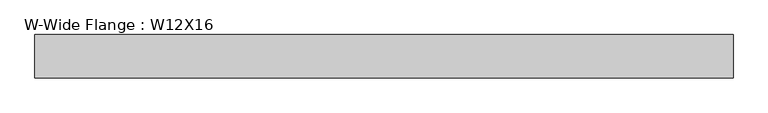
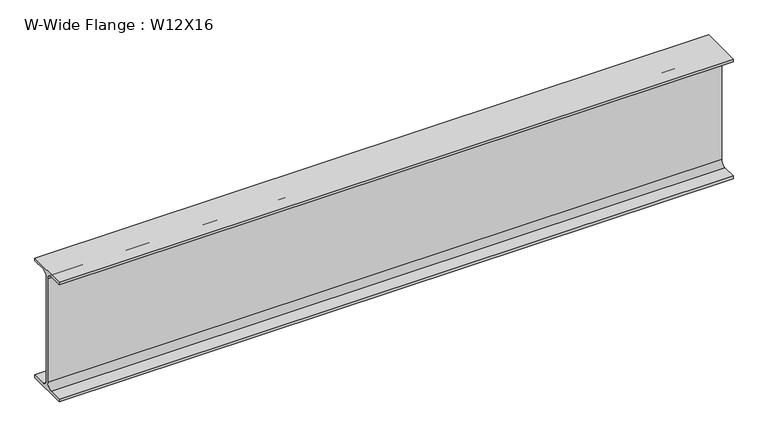
"""IFC4 building model written with IfcOpenShell, lengths in millimetres: beam geometry, W-Wide Flange : W12X16."""

from ifc_helpers import new_model, si_unit, point, frame, frame_2d, origin, place, context, project, spatial, polyline, circle_curve, trimmed, segment, composite_curve, outline, extrude, source, transform, mapped, element, save


def w_wide_flange_w12x16_6f895092(model_context):
    return source(origin(), model_context, "Body", "SweptSolid", [
        extrude(outline(composite_curve([segment(polyline([(50.673, -145.669), (50.673, -152.4), (-50.673, -152.4), (-50.673, -145.669), (-16.7005, -145.669)]), True, "CONTINUOUS"), segment(trimmed(circle_curve(frame_2d((-16.7005, -131.7625)), 13.9065), [point((-16.7005, -145.669))], [point((-2.794, -131.7625))], True, "CARTESIAN"), True, "CONTINUOUS"), segment(polyline([(-2.794, -131.7625), (-2.794, 131.7625)]), True, "CONTINUOUS"), segment(trimmed(circle_curve(frame_2d((-16.7005, 131.7625)), 13.9065), [point((-2.794, 131.7625))], [point((-16.7005, 145.669))], True, "CARTESIAN"), True, "CONTINUOUS"), segment(polyline([(-16.7005, 145.669), (-50.673, 145.669), (-50.673, 152.4), (50.673, 152.4), (50.673, 145.669), (16.7005, 145.669)]), True, "CONTINUOUS"), segment(trimmed(circle_curve(frame_2d((16.7005, 131.7625)), 13.9065), [point((16.7005, 145.669))], [point((2.794, 131.7625))], True, "CARTESIAN"), True, "CONTINUOUS"), segment(polyline([(2.794, 131.7625), (2.794, -131.7625)]), True, "CONTINUOUS"), segment(trimmed(circle_curve(frame_2d((16.7005, -131.7625)), 13.9065), [point((2.794, -131.7625))], [point((16.7005, -145.669))], True, "CARTESIAN"), True, "CONTINUOUS"), segment(polyline([(16.7005, -145.669), (50.673, -145.669)]), True, "CONTINUOUS")], self_intersect=False)), frame((-812.673, 0.0, 0.0), z_axis=(1.0, 0.0, 0.0), x_axis=(0.0, 1.0, 0.0)), (0.0, 0.0, 1.0), 1625.346),
    ])


if __name__ == "__main__":
    model = new_model("IFC4")
    model_context = context("Model", 3, world=origin())
    ifc_project = project(units=[si_unit("LENGTHUNIT", "METRE", prefix="MILLI")], contexts=[model_context])
    site = spatial("IfcSite", under=ifc_project)
    building = spatial("IfcBuilding", under=site)
    placement = place(None, origin())
    w_wide_flange_w12x16_shape = w_wide_flange_w12x16_6f895092(model_context)
    element("IfcBeam", 1, ObjectType="W-Wide Flange : W12X16", at=placement, inside=building, context=model_context, shape_type="MappedRepresentation", body=[
        mapped(w_wide_flange_w12x16_shape, transform((0.0, 0.0, 0.0), x_axis=(1.0, 0.0, 0.0), y_axis=(0.0, 1.0, 0.0), z_axis=(0.0, 0.0, 1.0))),
    ])
    save(model, "model.ifc")

# Revit data of these elements
# Type "W-Wide Flange : W12X16"
#   Assembly Code = "B10"
#   W = 16
#   Length [instance default] = 5' - 0"
#   bf = 0' - 3.99"
#   d = 1' - 0"
#   k = 0' - 0 13/16"
#   k2 = 0' - 0.5475"
#   tf = 0' - 0.265"
#   tw = 0' - 0.22"
#   A = 0.0327083 SF
#   Structural Material [instance default] = Steel ASTM A992
# Element 1 (IfcBeam, "W-Wide Flange : W12X16")
#   Structural Material = Steel ASTM A36
#   Materials on its faces: "Steel ASTM A36"
# Materials
#   "Steel ASTM A992": class "Metal", colour RGB 199 199 199, transparency 0, Description = "Structural steel 50ksi", Cost = 0
#   "Steel ASTM A36": class "Metal", colour RGB 199 199 199, transparency 0, Description = "Structural steel, ASTM A36 Grade B, mill finish", Cost = 0
